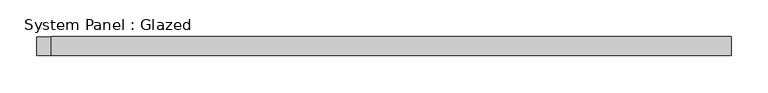
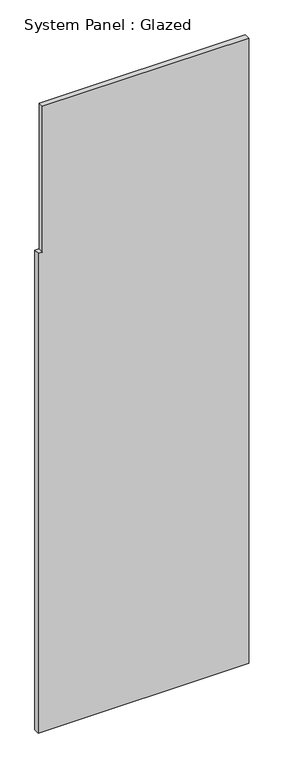
"""IFC4 building model written with IfcOpenShell, lengths in millimetres: plate geometry, System Panel : Glazed."""

import ifcopenshell
import ifcopenshell.guid

model = None  # the IFC model being written
_history = None  # IfcOwnerHistory: only IFC2X3 demands one
_inside = {}  # id of a spatial element -> (the spatial element, [elements in it])
_under = {}  # id of a project, library or spatial element -> (it, [spatial elements below it])
_declared = {}  # id of a project -> (the project, [libraries it declares])
_typed = {}  # id of a type object -> (the type object, [elements of that type])
_made_of = {}  # id of a material, layer set ... -> (it, [elements and type objects made of it])


def new_model(schema):
    """Start an empty IFC model of exactly this schema.

    Asked for "IFC4X3", IfcOpenShell would pick the latest addendum, in which some entities
    have other attributes; the version numbers below select the first issue.
    IFC2X3 requires an IfcOwnerHistory on every rooted entity: one is made here for all.
    """
    global model, _history
    if schema == "IFC4X3":
        model = ifcopenshell.file(schema_version=(4, 3, 0, 0))
    else:
        model = ifcopenshell.file(schema=schema)
    _inside.clear()
    _under.clear()
    _declared.clear()
    _typed.clear()
    _made_of.clear()
    _history = None
    if model.schema == "IFC2X3":
        org = make("IfcOrganization", Name="unknown")
        user = make(
            "IfcPersonAndOrganization",
            ThePerson=make("IfcPerson", FamilyName="unknown"),
            TheOrganization=org,
        )
        app = make(
            "IfcApplication",
            ApplicationDeveloper=org,
            Version="unknown",
            ApplicationFullName="unknown",
            ApplicationIdentifier="unknown",
        )
        _history = make(
            "IfcOwnerHistory",
            OwningUser=user,
            OwningApplication=app,
            ChangeAction="ADDED",
            CreationDate=0,
        )
    return model


def make(cls, **values):
    """One entity of the class cls with the attributes given. An attribute that is None is left unset."""
    return model.create_entity(
        cls, **{name: value for name, value in values.items() if value is not None}
    )


def rooted(cls, **values):
    """An entity with a GlobalId (a new one), such as an element, a storey or a relation."""
    return make(cls, GlobalId=ifcopenshell.guid.new(), OwnerHistory=_history, **values)


def si_unit(unit_type, name, prefix=None):
    """IfcSIUnit, for example si_unit("LENGTHUNIT", "METRE", prefix="MILLI")."""
    return make("IfcSIUnit", UnitType=unit_type, Prefix=prefix, Name=name)


def assignment(units):
    """IfcUnitAssignment: the units of a project."""
    return None if units is None else make("IfcUnitAssignment", Units=units)


def point(xyz):
    """IfcCartesianPoint."""
    return None if xyz is None else make("IfcCartesianPoint", Coordinates=xyz)


def direction(xyz):
    """IfcDirection."""
    return None if xyz is None else make("IfcDirection", DirectionRatios=xyz)


def frame(location, z_axis=None, x_axis=None):
    """IfcAxis2Placement3D, a coordinate frame: its origin and axes. An axis left out is left unset."""
    return make(
        "IfcAxis2Placement3D",
        Location=point(location),
        Axis=direction(z_axis),
        RefDirection=direction(x_axis),
    )


def origin():
    """The frame at (0, 0, 0) with its axes left unset."""
    return frame((0.0, 0.0, 0.0))


def place(relative_to, where):
    """IfcLocalPlacement: puts the frame where relative to a parent placement (None: the world)."""
    return make(
        "IfcLocalPlacement", PlacementRelTo=relative_to, RelativePlacement=where
    )


def context(
    kind, dimensions, precision=None, world=None, true_north=None, identifier=None
):
    """IfcGeometricRepresentationContext, for example the 3D "Model" context."""
    return make(
        "IfcGeometricRepresentationContext",
        ContextIdentifier=identifier,
        ContextType=kind,
        CoordinateSpaceDimension=dimensions,
        Precision=precision,
        WorldCoordinateSystem=world,
        TrueNorth=true_north,
    )


def project(units=None, contexts=None):
    """IfcProject with its units and contexts."""
    return rooted(
        "IfcProject",
        Name="project",
        RepresentationContexts=contexts,
        UnitsInContext=assignment(units),
    )


def spatial(cls, under=None, at=None, **own):
    """A site, building, storey or space (cls), placed at a placement, below another one or the project."""
    s = rooted(cls, ObjectPlacement=at, **own)
    if under is not None:
        _under.setdefault(under.id(), (under, []))[1].append(s)
    return s


def polyline(points):
    """IfcPolyline through the points."""
    return make("IfcPolyline", Points=[point(p) for p in points])


def outline(outer, holes=None, kind="AREA"):
    """IfcArbitraryClosedProfileDef: a profile drawn as a closed curve; with holes, ...WithVoids."""
    if holes is None:
        return make("IfcArbitraryClosedProfileDef", ProfileType=kind, OuterCurve=outer)
    return make(
        "IfcArbitraryProfileDefWithVoids",
        ProfileType=kind,
        OuterCurve=outer,
        InnerCurves=holes,
    )


def extrude(swept, where, along, depth):
    """IfcExtrudedAreaSolid: the profile swept, set in the frame where, extruded along a direction by depth."""
    return make(
        "IfcExtrudedAreaSolid",
        SweptArea=swept,
        Position=where,
        ExtrudedDirection=direction(along),
        Depth=depth,
    )


def shape(context_of_items, identifier, shape_type, items):
    """IfcShapeRepresentation: the items that make up one representation, for example the "Body"."""
    return make(
        "IfcShapeRepresentation",
        ContextOfItems=context_of_items,
        RepresentationIdentifier=identifier,
        RepresentationType=shape_type,
        Items=items,
    )


def source(mapping_origin, context_of_items, identifier, shape_type, items):
    """IfcRepresentationMap: a shape defined once, which mapped items show again and again."""
    return make(
        "IfcRepresentationMap",
        MappingOrigin=mapping_origin,
        MappedRepresentation=shape(context_of_items, identifier, shape_type, items),
    )


def transform(
    local_origin,
    x_axis=None,
    y_axis=None,
    z_axis=None,
    scale=None,
    scale2=None,
    scale3=None,
    uniform=True,
):
    """IfcCartesianTransformationOperator3D, or its non-uniform kind. x_axis, y_axis, z_axis: its Axis1, 2, 3."""
    if uniform:
        return make(
            "IfcCartesianTransformationOperator3D",
            Axis1=direction(x_axis),
            Axis2=direction(y_axis),
            LocalOrigin=point(local_origin),
            Scale=scale,
            Axis3=direction(z_axis),
        )
    return make(
        "IfcCartesianTransformationOperator3DnonUniform",
        Axis1=direction(x_axis),
        Axis2=direction(y_axis),
        LocalOrigin=point(local_origin),
        Scale=scale,
        Axis3=direction(z_axis),
        Scale2=scale2,
        Scale3=scale3,
    )


def mapped(mapping_source, mapping_target):
    """IfcMappedItem: shows the shape of a source again, moved by a transform."""
    return make(
        "IfcMappedItem", MappingSource=mapping_source, MappingTarget=mapping_target
    )


def made_of(thing, what):
    """Note that an element or type object is made of a material, layer set ...; save() writes the relation."""
    if what is not None:
        _made_of.setdefault(what.id(), (what, []))[1].append(thing)
    return thing


def element(
    cls,
    number,
    at=None,
    inside=None,
    cuts=None,
    type_object=None,
    material=None,
    context=None,
    identifier="Body",
    shape_type=None,
    held_by="IfcProductDefinitionShape",
    body=None,
    shapes=None,
    **own,
):
    """One element of the class cls, such as IfcWall. Its Tag is "e" and its number.

    at: its placement. inside: the storey or other place that contains it. cuts: it is an
    opening in that element (IfcRelVoidsElement). A single representation is given by context,
    identifier, shape_type and body (its items); several are given by shapes. held_by: the class
    of the entity that holds the representations. save() writes the other relations.
    """
    e = rooted(cls, Tag="e%d" % number, ObjectPlacement=at, **own)
    if body is not None:
        shapes = [shape(context, identifier, shape_type, body)]
    if shapes is not None:
        e.Representation = make(held_by, Representations=shapes)
    if inside is not None:
        _inside.setdefault(inside.id(), (inside, []))[1].append(e)
    if cuts is not None:
        rooted(
            "IfcRelVoidsElement", RelatingBuildingElement=cuts, RelatedOpeningElement=e
        )
    if type_object is not None:
        _typed.setdefault(type_object.id(), (type_object, []))[1].append(e)
    return made_of(e, material)


def aggregate(whole, parts):
    """IfcRelAggregates: a whole, such as a stair, and the parts it consists of."""
    return rooted("IfcRelAggregates", RelatingObject=whole, RelatedObjects=parts)


def save(model, path):
    """Write the relations noted so far, then the file.

    IfcRelAggregates (storeys below a building ...), IfcRelContainedInSpatialStructure (elements
    in a storey), IfcRelDefinesByType, IfcRelAssociatesMaterial and IfcRelDeclares: one each for
    every whole, place, type object, material and project.
    """
    for whole, parts in _under.values():
        aggregate(whole, parts)
    for where, things in _inside.values():
        rooted(
            "IfcRelContainedInSpatialStructure",
            RelatedElements=things,
            RelatingStructure=where,
        )
    for kind, things in _typed.values():
        rooted("IfcRelDefinesByType", RelatedObjects=things, RelatingType=kind)
    for what, things in _made_of.values():
        rooted("IfcRelAssociatesMaterial", RelatedObjects=things, RelatingMaterial=what)
    for by, libraries in _declared.values():
        rooted("IfcRelDeclares", RelatingContext=by, RelatedDefinitions=libraries)
    model.write(path)


def system_panel_glazed_1ffcdd07(model_context):
    return source(origin(), model_context, "Body", "SweptSolid", [
        extrude(outline(polyline([(0.0, -469.2560996), (0.0, 469.2560996), (2260.6, 469.2560996), (2946.4, 469.2560996), (2946.4, -450.2060996), (2260.6, -450.2060996), (2260.6, -469.2560996), (0.0, -469.2560996)])), frame((0.0, -12.7, 0.0), z_axis=(0.0, 1.0, 0.0), x_axis=(0.0, 0.0, 1.0)), (0.0, 0.0, 1.0), 25.4),
    ])


if __name__ == "__main__":
    model = new_model("IFC4")
    model_context = context("Model", 3, world=origin())
    ifc_project = project(units=[si_unit("LENGTHUNIT", "METRE", prefix="MILLI")], contexts=[model_context])
    site = spatial("IfcSite", under=ifc_project)
    building = spatial("IfcBuilding", under=site)
    placement = place(None, origin())
    system_panel_glazed_shape = system_panel_glazed_1ffcdd07(model_context)
    element("IfcPlate", 1, ObjectType="System Panel : Glazed", at=placement, inside=building, context=model_context, shape_type="MappedRepresentation", body=[
        mapped(system_panel_glazed_shape, transform((0.0, 0.0, 0.0), x_axis=(1.0, 0.0, 0.0), y_axis=(0.0, 1.0, 0.0), z_axis=(0.0, 0.0, 1.0))),
    ])
    save(model, "model.ifc")

# Revit data of these elements
# Element 1 (IfcPlate, "System Panel : Glazed")
#   Materials on its faces: "BUTT GLAZED STOREFRONT WITH VERTICAL MULLION"
# Materials
#   "BUTT GLAZED STOREFRONT WITH VERTICAL MULLION": class "Glass", colour RGB 236 240 239, transparency 0.39, Description = "Soda Lime Glass", Cost = 0
